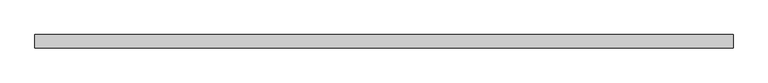
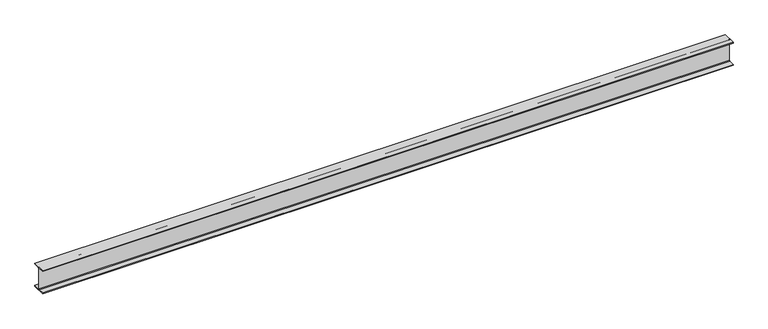
"""IFC4 building model written with IfcOpenShell, lengths in millimetres: beam geometry, Old_Steel Beam_H-KSD3502 : H_SB_ASB_H-350×175x7x11."""

import ifcopenshell
import ifcopenshell.guid

model = None  # the IFC model being written
_history = None  # IfcOwnerHistory: only IFC2X3 demands one
_inside = {}  # id of a spatial element -> (the spatial element, [elements in it])
_under = {}  # id of a project, library or spatial element -> (it, [spatial elements below it])
_declared = {}  # id of a project -> (the project, [libraries it declares])
_typed = {}  # id of a type object -> (the type object, [elements of that type])
_made_of = {}  # id of a material, layer set ... -> (it, [elements and type objects made of it])


def new_model(schema):
    """Start an empty IFC model of exactly this schema.

    Asked for "IFC4X3", IfcOpenShell would pick the latest addendum, in which some entities
    have other attributes; the version numbers below select the first issue.
    IFC2X3 requires an IfcOwnerHistory on every rooted entity: one is made here for all.
    """
    global model, _history
    if schema == "IFC4X3":
        model = ifcopenshell.file(schema_version=(4, 3, 0, 0))
    else:
        model = ifcopenshell.file(schema=schema)
    _inside.clear()
    _under.clear()
    _declared.clear()
    _typed.clear()
    _made_of.clear()
    _history = None
    if model.schema == "IFC2X3":
        org = make("IfcOrganization", Name="unknown")
        user = make(
            "IfcPersonAndOrganization",
            ThePerson=make("IfcPerson", FamilyName="unknown"),
            TheOrganization=org,
        )
        app = make(
            "IfcApplication",
            ApplicationDeveloper=org,
            Version="unknown",
            ApplicationFullName="unknown",
            ApplicationIdentifier="unknown",
        )
        _history = make(
            "IfcOwnerHistory",
            OwningUser=user,
            OwningApplication=app,
            ChangeAction="ADDED",
            CreationDate=0,
        )
    return model


def make(cls, **values):
    """One entity of the class cls with the attributes given. An attribute that is None is left unset."""
    return model.create_entity(
        cls, **{name: value for name, value in values.items() if value is not None}
    )


def rooted(cls, **values):
    """An entity with a GlobalId (a new one), such as an element, a storey or a relation."""
    return make(cls, GlobalId=ifcopenshell.guid.new(), OwnerHistory=_history, **values)


def si_unit(unit_type, name, prefix=None):
    """IfcSIUnit, for example si_unit("LENGTHUNIT", "METRE", prefix="MILLI")."""
    return make("IfcSIUnit", UnitType=unit_type, Prefix=prefix, Name=name)


def assignment(units):
    """IfcUnitAssignment: the units of a project."""
    return None if units is None else make("IfcUnitAssignment", Units=units)


def point(xyz):
    """IfcCartesianPoint."""
    return None if xyz is None else make("IfcCartesianPoint", Coordinates=xyz)


def direction(xyz):
    """IfcDirection."""
    return None if xyz is None else make("IfcDirection", DirectionRatios=xyz)


def frame(location, z_axis=None, x_axis=None):
    """IfcAxis2Placement3D, a coordinate frame: its origin and axes. An axis left out is left unset."""
    return make(
        "IfcAxis2Placement3D",
        Location=point(location),
        Axis=direction(z_axis),
        RefDirection=direction(x_axis),
    )


def frame_2d(location, x_axis=None):
    """IfcAxis2Placement2D, a coordinate frame in the plane: its origin and x axis."""
    return make(
        "IfcAxis2Placement2D", Location=point(location), RefDirection=direction(x_axis)
    )


def origin():
    """The frame at (0, 0, 0) with its axes left unset."""
    return frame((0.0, 0.0, 0.0))


def place(relative_to, where):
    """IfcLocalPlacement: puts the frame where relative to a parent placement (None: the world)."""
    return make(
        "IfcLocalPlacement", PlacementRelTo=relative_to, RelativePlacement=where
    )


def context(
    kind, dimensions, precision=None, world=None, true_north=None, identifier=None
):
    """IfcGeometricRepresentationContext, for example the 3D "Model" context."""
    return make(
        "IfcGeometricRepresentationContext",
        ContextIdentifier=identifier,
        ContextType=kind,
        CoordinateSpaceDimension=dimensions,
        Precision=precision,
        WorldCoordinateSystem=world,
        TrueNorth=true_north,
    )


def project(units=None, contexts=None):
    """IfcProject with its units and contexts."""
    return rooted(
        "IfcProject",
        Name="project",
        RepresentationContexts=contexts,
        UnitsInContext=assignment(units),
    )


def spatial(cls, under=None, at=None, **own):
    """A site, building, storey or space (cls), placed at a placement, below another one or the project."""
    s = rooted(cls, ObjectPlacement=at, **own)
    if under is not None:
        _under.setdefault(under.id(), (under, []))[1].append(s)
    return s


def polyline(points):
    """IfcPolyline through the points."""
    return make("IfcPolyline", Points=[point(p) for p in points])


def circle_curve(where, radius):
    """IfcCircle in the frame where."""
    return make("IfcCircle", Position=where, Radius=radius)


def trimmed(basis, trim1, trim2, sense, master):
    """IfcTrimmedCurve: the piece of a basis curve between two trims."""
    return make(
        "IfcTrimmedCurve",
        BasisCurve=basis,
        Trim1=trim1,
        Trim2=trim2,
        SenseAgreement=sense,
        MasterRepresentation=master,
    )


def segment(curve, same_sense, transition):
    """IfcCompositeCurveSegment."""
    return make(
        "IfcCompositeCurveSegment",
        Transition=transition,
        SameSense=same_sense,
        ParentCurve=curve,
    )


def composite_curve(segments, self_intersect=None):
    """IfcCompositeCurve: segments joined end to end."""
    return make("IfcCompositeCurve", Segments=segments, SelfIntersect=self_intersect)


def outline(outer, holes=None, kind="AREA"):
    """IfcArbitraryClosedProfileDef: a profile drawn as a closed curve; with holes, ...WithVoids."""
    if holes is None:
        return make("IfcArbitraryClosedProfileDef", ProfileType=kind, OuterCurve=outer)
    return make(
        "IfcArbitraryProfileDefWithVoids",
        ProfileType=kind,
        OuterCurve=outer,
        InnerCurves=holes,
    )


def extrude(swept, where, along, depth):
    """IfcExtrudedAreaSolid: the profile swept, set in the frame where, extruded along a direction by depth."""
    return make(
        "IfcExtrudedAreaSolid",
        SweptArea=swept,
        Position=where,
        ExtrudedDirection=direction(along),
        Depth=depth,
    )


def shape(context_of_items, identifier, shape_type, items):
    """IfcShapeRepresentation: the items that make up one representation, for example the "Body"."""
    return make(
        "IfcShapeRepresentation",
        ContextOfItems=context_of_items,
        RepresentationIdentifier=identifier,
        RepresentationType=shape_type,
        Items=items,
    )


def source(mapping_origin, context_of_items, identifier, shape_type, items):
    """IfcRepresentationMap: a shape defined once, which mapped items show again and again."""
    return make(
        "IfcRepresentationMap",
        MappingOrigin=mapping_origin,
        MappedRepresentation=shape(context_of_items, identifier, shape_type, items),
    )


def transform(
    local_origin,
    x_axis=None,
    y_axis=None,
    z_axis=None,
    scale=None,
    scale2=None,
    scale3=None,
    uniform=True,
):
    """IfcCartesianTransformationOperator3D, or its non-uniform kind. x_axis, y_axis, z_axis: its Axis1, 2, 3."""
    if uniform:
        return make(
            "IfcCartesianTransformationOperator3D",
            Axis1=direction(x_axis),
            Axis2=direction(y_axis),
            LocalOrigin=point(local_origin),
            Scale=scale,
            Axis3=direction(z_axis),
        )
    return make(
        "IfcCartesianTransformationOperator3DnonUniform",
        Axis1=direction(x_axis),
        Axis2=direction(y_axis),
        LocalOrigin=point(local_origin),
        Scale=scale,
        Axis3=direction(z_axis),
        Scale2=scale2,
        Scale3=scale3,
    )


def mapped(mapping_source, mapping_target):
    """IfcMappedItem: shows the shape of a source again, moved by a transform."""
    return make(
        "IfcMappedItem", MappingSource=mapping_source, MappingTarget=mapping_target
    )


def made_of(thing, what):
    """Note that an element or type object is made of a material, layer set ...; save() writes the relation."""
    if what is not None:
        _made_of.setdefault(what.id(), (what, []))[1].append(thing)
    return thing


def element(
    cls,
    number,
    at=None,
    inside=None,
    cuts=None,
    type_object=None,
    material=None,
    context=None,
    identifier="Body",
    shape_type=None,
    held_by="IfcProductDefinitionShape",
    body=None,
    shapes=None,
    **own,
):
    """One element of the class cls, such as IfcWall. Its Tag is "e" and its number.

    at: its placement. inside: the storey or other place that contains it. cuts: it is an
    opening in that element (IfcRelVoidsElement). A single representation is given by context,
    identifier, shape_type and body (its items); several are given by shapes. held_by: the class
    of the entity that holds the representations. save() writes the other relations.
    """
    e = rooted(cls, Tag="e%d" % number, ObjectPlacement=at, **own)
    if body is not None:
        shapes = [shape(context, identifier, shape_type, body)]
    if shapes is not None:
        e.Representation = make(held_by, Representations=shapes)
    if inside is not None:
        _inside.setdefault(inside.id(), (inside, []))[1].append(e)
    if cuts is not None:
        rooted(
            "IfcRelVoidsElement", RelatingBuildingElement=cuts, RelatedOpeningElement=e
        )
    if type_object is not None:
        _typed.setdefault(type_object.id(), (type_object, []))[1].append(e)
    return made_of(e, material)


def aggregate(whole, parts):
    """IfcRelAggregates: a whole, such as a stair, and the parts it consists of."""
    return rooted("IfcRelAggregates", RelatingObject=whole, RelatedObjects=parts)


def save(model, path):
    """Write the relations noted so far, then the file.

    IfcRelAggregates (storeys below a building ...), IfcRelContainedInSpatialStructure (elements
    in a storey), IfcRelDefinesByType, IfcRelAssociatesMaterial and IfcRelDeclares: one each for
    every whole, place, type object, material and project.
    """
    for whole, parts in _under.values():
        aggregate(whole, parts)
    for where, things in _inside.values():
        rooted(
            "IfcRelContainedInSpatialStructure",
            RelatedElements=things,
            RelatingStructure=where,
        )
    for kind, things in _typed.values():
        rooted("IfcRelDefinesByType", RelatedObjects=things, RelatingType=kind)
    for what, things in _made_of.values():
        rooted("IfcRelAssociatesMaterial", RelatedObjects=things, RelatingMaterial=what)
    for by, libraries in _declared.values():
        rooted("IfcRelDeclares", RelatingContext=by, RelatedDefinitions=libraries)
    model.write(path)


def beam_6852f715(model_context):
    return source(origin(), model_context, "Body", "SweptSolid", [
        extrude(outline(composite_curve([segment(polyline([(82.5, -141.5), (82.5, -151.7), (-82.5, -151.7), (-82.5, -141.5), (-11.9, -141.5)]), True, "CONTINUOUS"), segment(trimmed(circle_curve(frame_2d((-11.9, -132.6)), 8.9), [point((-11.9, -141.5))], [point((-3.0, -132.6))], True, "CARTESIAN"), True, "CONTINUOUS"), segment(polyline([(-3.0, -132.6), (-3.0, 132.6)]), True, "CONTINUOUS"), segment(trimmed(circle_curve(frame_2d((-11.9, 132.6)), 8.9), [point((-3.0, 132.6))], [point((-11.9, 141.5))], True, "CARTESIAN"), True, "CONTINUOUS"), segment(polyline([(-11.9, 141.5), (-82.5, 141.5), (-82.5, 151.7), (82.5, 151.7), (82.5, 141.5), (11.9, 141.5)]), True, "CONTINUOUS"), segment(trimmed(circle_curve(frame_2d((11.9, 132.6)), 8.9), [point((11.9, 141.5))], [point((3.0, 132.6))], True, "CARTESIAN"), True, "CONTINUOUS"), segment(polyline([(3.0, 132.6), (3.0, -132.6)]), True, "CONTINUOUS"), segment(trimmed(circle_curve(frame_2d((11.9, -132.6)), 8.9), [point((3.0, -132.6))], [point((11.9, -141.5))], True, "CARTESIAN"), True, "CONTINUOUS"), segment(polyline([(11.9, -141.5), (82.5, -141.5)]), True, "CONTINUOUS")], self_intersect=False)), frame((-4298.8712061, 0.0, 0.0), z_axis=(1.0, 0.0, 0.0), x_axis=(0.0, 1.0, 0.0)), (0.0, 0.0, 1.0), 8634.4837274),
    ])


if __name__ == "__main__":
    model = new_model("IFC4")
    model_context = context("Model", 3, world=origin())
    ifc_project = project(units=[si_unit("LENGTHUNIT", "METRE", prefix="MILLI")], contexts=[model_context])
    site = spatial("IfcSite", under=ifc_project)
    building = spatial("IfcBuilding", under=site)
    placement = place(None, origin())
    beam_shape = beam_6852f715(model_context)
    element("IfcBeam", 1, ObjectType="Old_Steel Beam_H-KSD3502 : H_SB_ASB_H-350×175x7x11", at=placement, inside=building, context=model_context, shape_type="MappedRepresentation", body=[
        mapped(beam_shape, transform((0.0, 0.0, 0.0), x_axis=(1.0, 0.0, 0.0), y_axis=(0.0, 1.0, 0.0), z_axis=(0.0, 0.0, 1.0))),
    ])
    save(model, "model.ifc")

# Revit data of these elements
# Type "Old_Steel Beam_H-KSD3502 : H_SB_ASB_H-350×175x7x11"
#   Width = 17.5 cm
#   Web Thickness = 0.7 cm
#   Web Fillet = 1.4 cm
#   Warping Constant = 282290.0 cm⁶
#   Torsional Moment of Inertia = 19.4042 cm⁴
#   Torsional Modulus = 1.0 cm³
#   Section Area = 63.14 cm²
#   Plastic Modulus weak axis = 174.0 cm³
#   Plastic Modulus strong axis = 868.0 cm³
#   Perimeter = 1.36 m²/m
#   Nominal Weight = 49.60 kgf/m
#   Moment of Inertia weak axis = 984.00 cm⁴
#   Moment of Inertia strong axis = 13600.00 cm⁴
#   Height = 35.0 cm
#   Flange Thickness = 1.1 cm
#   Elastic Modulus weak axis = 112.0 cm³
#   Elastic Modulus strong axis = 775.0 cm³
#   Centroid Vertical = 17.5 cm
#   Centroid Horizontal = 8.75 cm
#   Length [instance default] = 1.5240 m
#   Structural Material [instance default] = Steel, 45-345
#   Assembly Code = ""
# Element 1 (IfcBeam, "Old_Steel Beam_H-KSD3502 : H_SB_ASB_H-350×175x7x11")
#   Structural Material = none
# Materials
#   "Steel, 45-345": class "Metal", colour RGB 189 187 185, transparency 0, Description = "Steel 345 MPa", Cost = 0
